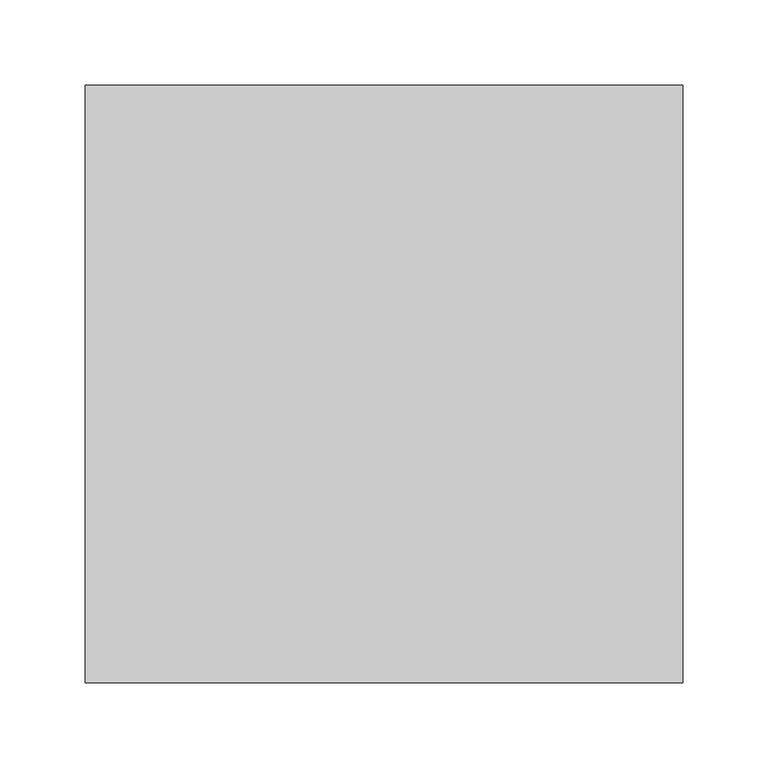
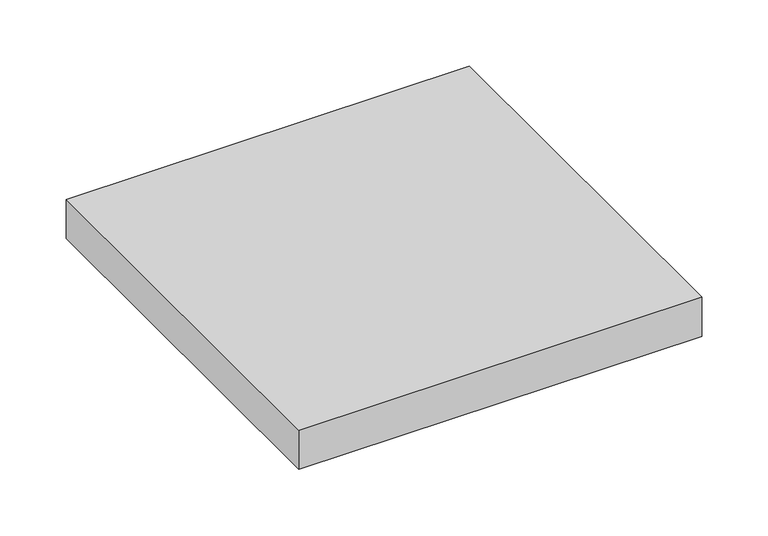
"""IFC4 building model written with IfcOpenShell, lengths in millimetres: proxy geometry, 플레이트18 : 플레이트."""

from ifc_helpers import new_model, si_unit, frame, origin, place, context, project, spatial, polyline, outline, extrude, source, transform, mapped, element, save


def generic_models_22d8b4c3(model_context):
    return source(origin(), model_context, "Body", "SweptSolid", [
        extrude(outline(polyline([(25169.0, 25924.5208589), (25169.0, 25574.5208589), (24819.0, 25574.5208589), (24819.0, 25924.5208589), (25169.0, 25924.5208589)])), frame((0.0, 0.0, 863.9720055), z_axis=(0.0, 0.0, 1.0), x_axis=(1.0, 0.0, 0.0)), (0.0, 0.0, 1.0), 36.0),
    ])


if __name__ == "__main__":
    model = new_model("IFC4")
    model_context = context("Model", 3, world=origin())
    ifc_project = project(units=[si_unit("LENGTHUNIT", "METRE", prefix="MILLI")], contexts=[model_context])
    site = spatial("IfcSite", under=ifc_project)
    building = spatial("IfcBuilding", under=site)
    placement = place(None, origin())
    generic_models_shape = generic_models_22d8b4c3(model_context)
    element("IfcBuildingElementProxy", 1, Name="플레이트18 : 플레이트", ObjectType="플레이트18 : 플레이트", at=placement, inside=building, context=model_context, shape_type="MappedRepresentation", body=[
        mapped(generic_models_shape, transform((0.0, 0.0, 0.0), x_axis=(1.0, 0.0, 0.0), y_axis=(0.0, 1.0, 0.0), z_axis=(0.0, 0.0, 1.0))),
    ])
    save(model, "model.ifc")
